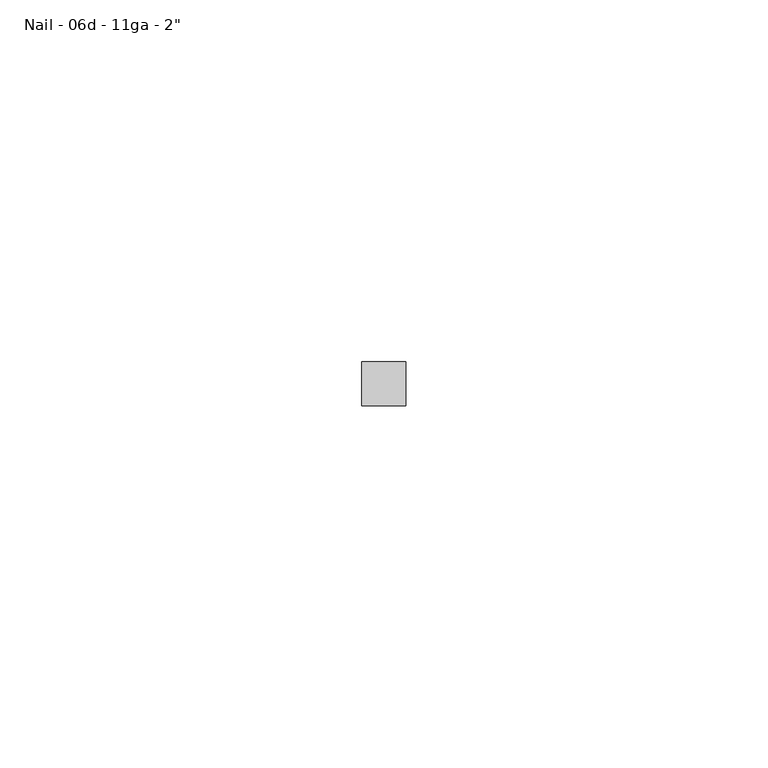
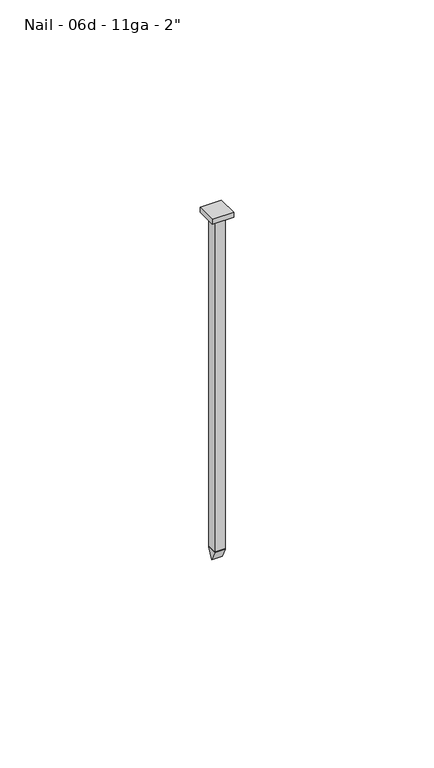
"""IFC4 building model written with IfcOpenShell, lengths in millimetres: fastener geometry."""

from ifc_helpers import new_model, si_unit, frame, origin, origin_with_axes, place, context, project, spatial, polyline, outline, extrude, source, transform, mapped, element, save


def fastener_eca79e8d(model_context):
    return source(origin(), model_context, "Body", "SweptSolid", [
        extrude(outline(polyline([(0.0, -104.648), (-1.524, -101.6), (1.524, -101.6), (0.0, -104.648)])), frame((-1.524, 0.0, 0.0), z_axis=(1.0, 0.0, 0.0), x_axis=(0.0, 1.0, 0.0)), (0.0, 0.0, 1.0), 3.048),
        extrude(outline(polyline([(-3.048, -3.048), (-3.048, 3.048), (3.048, 3.048), (3.048, -3.048), (-3.048, -3.048)])), origin_with_axes(), (0.0, 0.0, 1.0), 1.524),
        extrude(outline(polyline([(-1.524, 1.524), (1.524, 1.524), (1.524, -1.524), (-1.524, -1.524), (-1.524, 1.524)])), frame((0.0, 0.0, -101.6), z_axis=(0.0, 0.0, 1.0), x_axis=(1.0, 0.0, 0.0)), (0.0, 0.0, 1.0), 101.6),
    ])


if __name__ == "__main__":
    model = new_model("IFC4")
    model_context = context("Model", 3, world=origin())
    ifc_project = project(units=[si_unit("LENGTHUNIT", "METRE", prefix="MILLI")], contexts=[model_context])
    site = spatial("IfcSite", under=ifc_project)
    building = spatial("IfcBuilding", under=site)
    placement = place(None, origin())
    fastener_shape = fastener_eca79e8d(model_context)
    element("IfcFastener", 1, ObjectType="060523 - W_P_C - Fastenings - Generic - SQUARE : Nail - 06d - 11ga - 2\"", at=placement, inside=building, context=model_context, shape_type="MappedRepresentation", body=[
        mapped(fastener_shape, transform((0.0, 0.0, 0.0), x_axis=(1.0, 0.0, 0.0), y_axis=(0.0, 1.0, 0.0), z_axis=(0.0, 0.0, 1.0))),
    ])
    save(model, "model.ifc")

# Revit data of these elements
# Type "060523 - W_P_C - Fastenings - Generic - SQUARE : Nail - 06d - 11ga - 2\""
#   Washer_Thickness = 0' - 0.00333"
#   Washer Radius = 0' - 0.07"
#   Washer Offset - Head = 0' - 0"
#   Washer Offset = 0' - 0"
#   Thickness_of_Substrate [instance default] = 0' - 1"
#   Side = 0' - 0 37/64"
#   Radius = 0' - 0.06"
#   Length [instance default] = 0' - 2"
#   Head Size = 0' - 1"
#   Head Radius = 0' - 0 1/2"
#   Head Height = 0' - 0.01"
#   Double Diameter = 0' - 0.24"
#   Diameter = 0' - 0.12"
#   Default Elevation = 4' - 0"
#   Washer_Nut_Visibility = no
#   Washer_Head_Visibility = no
#   Round_Head_Visibility = yes
#   Point Visibility = yes
#   Nut_Visibility = no
#   Hex_Head_Visiblilty = no
#   Washer Material = none
#   Bolt Material (Size) = AT SILL - FASTENER AT 24" O.C.
# Element 1 (IfcFastener, "060523 - W_P_C - Fastenings - Generic - SQUARE : Nail - 06d - 11ga - 2\"")
#   Length = 0' - 4"
# Materials
#   "AT SILL - FASTENER AT 24\" O.C.": class "Generic", colour RGB 120 120 120, transparency 0, Cost = 0
